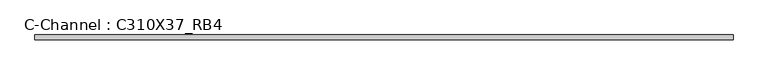
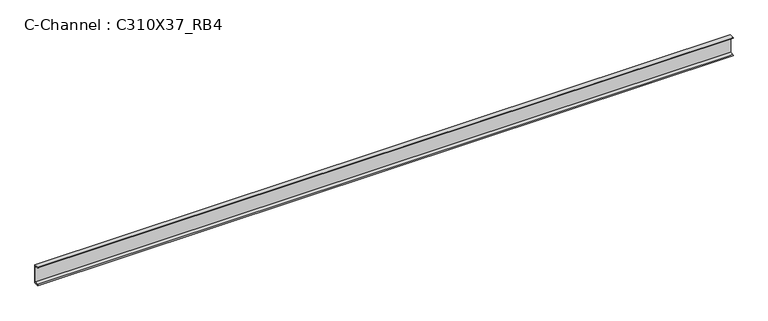
"""IFC4 building model written with IfcOpenShell, lengths in millimetres: beam geometry, C-Channel : C310X37_RB4."""

from ifc_helpers import new_model, si_unit, point, frame, frame_2d, origin, place, context, project, spatial, polyline, circle_curve, trimmed, segment, composite_curve, outline, extrude, source, transform, mapped, element, save


def c_channel_c310x37_rb4_fb7ce729(model_context):
    return source(origin(), model_context, "Body", "SweptSolid", [
        extrude(outline(composite_curve([segment(polyline([(17.1196, 152.4), (17.1196, -152.4), (-60.3504, -152.4)]), True, "CONTINUOUS"), segment(trimmed(circle_curve(frame_2d((-47.625, -152.4)), 12.7254), [point((-60.3504, -152.4))], [point((-47.625, -139.6746))], False, "CARTESIAN"), True, "CONTINUOUS"), segment(polyline([(-47.625, -139.6746), (7.2898, -130.9769501), (7.2898, 130.9769501), (-47.625, 139.6746)]), True, "CONTINUOUS"), segment(trimmed(circle_curve(frame_2d((-47.625, 152.4)), 12.7254), [point((-47.625, 139.6746))], [point((-60.3504, 152.4))], False, "CARTESIAN"), True, "CONTINUOUS"), segment(polyline([(-60.3504, 152.4), (17.1196, 152.4)]), True, "CONTINUOUS")], self_intersect=False)), frame((-5538.3209452, 0.0, 0.0), z_axis=(1.0, 0.0, 0.0), x_axis=(0.0, 1.0, 0.0)), (0.0, 0.0, 1.0), 11055.4234616),
    ])


if __name__ == "__main__":
    model = new_model("IFC4")
    model_context = context("Model", 3, world=origin())
    ifc_project = project(units=[si_unit("LENGTHUNIT", "METRE", prefix="MILLI")], contexts=[model_context])
    site = spatial("IfcSite", under=ifc_project)
    building = spatial("IfcBuilding", under=site)
    placement = place(None, origin())
    c_channel_c310x37_rb4_shape = c_channel_c310x37_rb4_fb7ce729(model_context)
    element("IfcBeam", 1, ObjectType="C-Channel : C310X37_RB4", at=placement, inside=building, context=model_context, shape_type="MappedRepresentation", body=[
        mapped(c_channel_c310x37_rb4_shape, transform((0.0, 0.0, 0.0), x_axis=(1.0, 0.0, 0.0), y_axis=(0.0, 1.0, 0.0), z_axis=(0.0, 0.0, 1.0))),
    ])
    save(model, "model.ifc")

# Revit data of these elements
# Type "C-Channel : C310X37_RB4"
#   Assembly Code = "B10"
#   W = 25
#   Length [instance default] = 1524 mm
#   bf = 77.47 mm
#   d = 304.8 mm
#   tf = 12.725 mm
#   tw = 9.83 mm
#   x = 17.12 mm
#   A = 0.00473547 m²
#   Structural Material [instance default] = Steel ASTM A36
# Element 1 (IfcBeam, "C-Channel : C310X37_RB4")
#   Structural Material = Steel ASTM A992
#   Materials on its faces: "Steel ASTM A992"
# Materials
#   "Steel ASTM A36": class "Metal", colour RGB 199 199 199, transparency 0, Description = "Structural steel, ASTM A36 Grade B, mill finish", Cost = 0
#   "Steel ASTM A992": class "Metal", colour RGB 199 199 199, transparency 0, Description = "Structural steel 50ksi", Cost = 0
